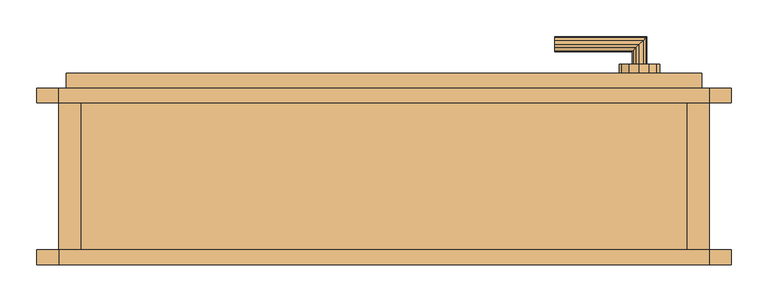
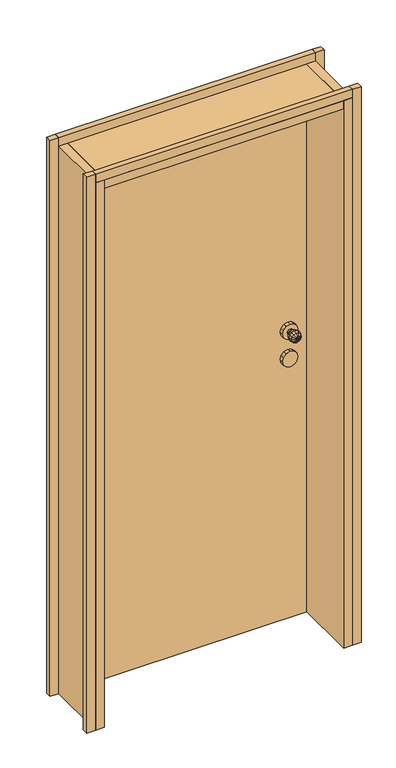
"""IFC4 building model written with IfcOpenShell, lengths in millimetres: door geometry, Tür."""

from ifc_helpers import new_model, si_unit, frame, origin, place, context, project, spatial, polyline, outline, extrude, faceted_brep, source, transform, mapped, element, save


def door_29abe8a6(model_context):
    return source(origin(), model_context, "Body", "SolidModel", [
        extrude(outline(polyline([(885.0, 220.0), (885.0, -20.0), (855.0, -20.0), (855.0, 220.0), (885.0, 220.0)])), frame((0.0, 0.0, 140.0), z_axis=(0.0, 0.0, 1.0), x_axis=(1.0, 0.0, 0.0)), (0.0, 0.0, 1.0), 1995.0),
        extrude(outline(polyline([(1176.25, 813.8156986), (1190.0, 817.5), (1203.75, 813.8156986), (1213.8156986, 803.75), (1217.5, 790.0), (1213.8156986, 776.25), (1203.75, 766.1843014), (1190.0, 762.5), (1176.25, 766.1843014), (1166.1843014, 776.25), (1162.5, 790.0), (1166.1843014, 803.75), (1176.25, 813.8156986)])), frame((0.0, 187.5, 0.0), z_axis=(0.0, 1.0, 0.0), x_axis=(0.0, 0.0, 1.0)), (0.0, 0.0, 1.0), 12.5),
        faceted_brep([(807.3205081, 150.0, 1190.0), (810.0, 160.0, 1190.0), (807.3205081, 160.0, 1200.0), (805.0, 150.0, 1198.660254), (800.0, 160.0, 1207.3205081), (798.660254, 150.0, 1205.0), (790.0, 160.0, 1210.0), (790.0, 150.0, 1207.3205081), (780.0, 160.0, 1207.3205081), (781.339746, 150.0, 1205.0), (772.6794919, 160.0, 1200.0), (775.0, 150.0, 1198.660254), (770.0, 160.0, 1190.0), (772.6794919, 150.0, 1190.0), (772.6794919, 160.0, 1180.0), (775.0, 150.0, 1181.339746), (780.0, 160.0, 1172.6794919), (781.339746, 150.0, 1175.0), (790.0, 160.0, 1170.0), (790.0, 150.0, 1172.6794919), (800.0, 160.0, 1172.6794919), (798.660254, 150.0, 1175.0), (807.3205081, 160.0, 1180.0), (805.0, 150.0, 1181.339746), (800.0, 142.6794919, 1190.0), (798.660254, 142.6794919, 1195.0), (795.0, 142.6794919, 1198.660254), (790.0, 142.6794919, 1200.0), (785.0, 142.6794919, 1198.660254), (781.339746, 142.6794919, 1195.0), (780.0, 142.6794919, 1190.0), (781.339746, 142.6794919, 1185.0), (785.0, 142.6794919, 1181.339746), (790.0, 142.6794919, 1180.0), (795.0, 142.6794919, 1181.339746), (798.660254, 142.6794919, 1185.0), (790.0, 140.0, 1190.0), (807.3205081, 170.0, 1190.0), (805.0, 170.0, 1198.660254), (798.660254, 170.0, 1205.0), (790.0, 170.0, 1207.3205081), (781.339746, 170.0, 1205.0), (775.0, 170.0, 1198.660254), (772.6794919, 170.0, 1190.0), (775.0, 170.0, 1181.339746), (781.339746, 170.0, 1175.0), (790.0, 170.0, 1172.6794919), (798.660254, 170.0, 1175.0), (805.0, 170.0, 1181.339746), (800.0, 177.3205081, 1190.0), (798.660254, 177.3205081, 1195.0), (795.0, 177.3205081, 1198.660254), (790.0, 177.3205081, 1200.0), (785.0, 177.3205081, 1198.660254), (781.339746, 177.3205081, 1195.0), (780.0, 177.3205081, 1190.0), (781.339746, 177.3205081, 1185.0), (785.0, 177.3205081, 1181.339746), (790.0, 177.3205081, 1180.0), (795.0, 177.3205081, 1181.339746), (798.660254, 177.3205081, 1185.0), (790.0, 180.0, 1190.0)], [[[0, 1, 2, 3]], [[3, 2, 4, 5]], [[5, 4, 6, 7]], [[7, 6, 8, 9]], [[9, 8, 10, 11]], [[11, 10, 12, 13]], [[13, 12, 14, 15]], [[15, 14, 16, 17]], [[17, 16, 18, 19]], [[19, 18, 20, 21]], [[21, 20, 22, 23]], [[23, 22, 1, 0]], [[24, 0, 3, 25]], [[25, 3, 5, 26]], [[26, 5, 7, 27]], [[27, 7, 9, 28]], [[28, 9, 11, 29]], [[29, 11, 13, 30]], [[30, 13, 15, 31]], [[31, 15, 17, 32]], [[32, 17, 19, 33]], [[33, 19, 21, 34]], [[34, 21, 23, 35]], [[35, 23, 0, 24]], [[36, 24, 25]], [[36, 25, 26]], [[36, 26, 27]], [[36, 27, 28]], [[36, 28, 29]], [[36, 29, 30]], [[36, 30, 31]], [[36, 31, 32]], [[36, 32, 33]], [[36, 33, 34]], [[36, 34, 35]], [[36, 35, 24]], [[1, 37, 38, 2]], [[2, 38, 39, 4]], [[4, 39, 40, 6]], [[6, 40, 41, 8]], [[8, 41, 42, 10]], [[10, 42, 43, 12]], [[12, 43, 44, 14]], [[14, 44, 45, 16]], [[16, 45, 46, 18]], [[18, 46, 47, 20]], [[20, 47, 48, 22]], [[22, 48, 37, 1]], [[37, 49, 50, 38]], [[38, 50, 51, 39]], [[39, 51, 52, 40]], [[40, 52, 53, 41]], [[41, 53, 54, 42]], [[42, 54, 55, 43]], [[43, 55, 56, 44]], [[44, 56, 57, 45]], [[45, 57, 58, 46]], [[46, 58, 59, 47]], [[47, 59, 60, 48]], [[48, 60, 49, 37]], [[49, 61, 50]], [[50, 61, 51]], [[51, 61, 52]], [[52, 61, 53]], [[53, 61, 54]], [[54, 61, 55]], [[55, 61, 56]], [[56, 61, 57]], [[57, 61, 58]], [[58, 61, 59]], [[59, 61, 60]], [[60, 61, 49]]]),
        extrude(outline(polyline([(1185.0, 798.660254), (1190.0, 800.0), (1195.0, 798.660254), (1198.660254, 795.0), (1200.0, 790.0), (1198.660254, 785.0), (1195.0, 781.339746), (1190.0, 780.0), (1185.0, 781.339746), (1181.339746, 785.0), (1180.0, 790.0), (1181.339746, 795.0), (1185.0, 798.660254)])), frame((0.0, 160.0, 0.0), z_axis=(0.0, 1.0, 0.0), x_axis=(0.0, 0.0, 1.0)), (0.0, 0.0, 1.0), 40.0),
        extrude(outline(polyline([(1066.1843014, 803.75), (1076.25, 813.8156986), (1090.0, 817.5), (1103.75, 813.8156986), (1113.8156986, 803.75), (1117.5, 790.0), (1113.8156986, 776.25), (1103.75, 766.1843014), (1090.0, 762.5), (1076.25, 766.1843014), (1066.1843014, 776.25), (1062.5, 790.0), (1066.1843014, 803.75)])), frame((0.0, 240.0, 0.0), z_axis=(0.0, 1.0, 0.0), x_axis=(0.0, 0.0, 1.0)), (0.0, 0.0, 1.0), 12.5),
        extrude(outline(polyline([(1076.25, 813.8156986), (1090.0, 817.5), (1103.75, 813.8156986), (1113.8156986, 803.75), (1117.5, 790.0), (1113.8156986, 776.25), (1103.75, 766.1843014), (1090.0, 762.5), (1076.25, 766.1843014), (1066.1843014, 776.25), (1062.5, 790.0), (1066.1843014, 803.75), (1076.25, 813.8156986)])), frame((0.0, 187.5, 0.0), z_axis=(0.0, 1.0, 0.0), x_axis=(0.0, 0.0, 1.0)), (0.0, 0.0, 1.0), 12.5),
        extrude(outline(polyline([(885.0, 220.0), (885.0, 200.0), (0.0, 200.0), (0.0, 220.0), (885.0, 220.0)])), frame((0.0, 0.0, 2135.0), z_axis=(0.0, 0.0, 1.0), x_axis=(1.0, 0.0, 0.0)), (0.0, 0.0, 1.0), 30.0),
        extrude(outline(polyline([(0.0, -20.0), (-30.0, -20.0), (-30.0, 0.0), (0.0, 0.0), (0.0, -20.0)])), frame((0.0, 0.0, 140.0), z_axis=(0.0, 0.0, 1.0), x_axis=(1.0, 0.0, 0.0)), (0.0, 0.0, 1.0), 2025.0),
        extrude(outline(polyline([(885.0, 0.0), (885.0, -20.0), (0.0, -20.0), (0.0, 0.0), (885.0, 0.0)])), frame((0.0, 0.0, 2135.0), z_axis=(0.0, 0.0, 1.0), x_axis=(1.0, 0.0, 0.0)), (0.0, 0.0, 1.0), 30.0),
        extrude(outline(polyline([(1166.1843014, 803.75), (1176.25, 813.8156986), (1190.0, 817.5), (1203.75, 813.8156986), (1213.8156986, 803.75), (1217.5, 790.0), (1213.8156986, 776.25), (1203.75, 766.1843014), (1190.0, 762.5), (1176.25, 766.1843014), (1166.1843014, 776.25), (1162.5, 790.0), (1166.1843014, 803.75)])), frame((0.0, 240.0, 0.0), z_axis=(0.0, 1.0, 0.0), x_axis=(0.0, 0.0, 1.0)), (0.0, 0.0, 1.0), 12.5),
        faceted_brep([(795.0, 240.0, 1198.660254), (790.0, 240.0, 1200.0), (785.0, 240.0, 1198.660254), (781.339746, 240.0, 1195.0), (780.0, 240.0, 1190.0), (781.339746, 240.0, 1185.0), (785.0, 240.0, 1181.339746), (790.0, 240.0, 1180.0), (795.0, 240.0, 1181.339746), (798.660254, 240.0, 1185.0), (800.0, 240.0, 1190.0), (798.660254, 240.0, 1195.0), (790.0, 280.0, 1200.0), (795.0, 285.0, 1198.660254), (798.660254, 288.660254, 1195.0), (800.0, 290.0, 1190.0), (798.660254, 288.660254, 1185.0), (795.0, 285.0, 1181.339746), (790.0, 280.0, 1180.0), (785.0, 275.0, 1181.339746), (781.339746, 271.339746, 1185.0), (780.0, 270.0, 1190.0), (781.339746, 271.339746, 1195.0), (785.0, 275.0, 1198.660254), (675.0, 275.0, 1198.660254), (675.0, 280.0, 1200.0), (675.0, 285.0, 1198.660254), (675.0, 288.660254, 1195.0), (675.0, 290.0, 1190.0), (675.0, 288.660254, 1185.0), (675.0, 285.0, 1181.339746), (675.0, 280.0, 1180.0), (675.0, 275.0, 1181.339746), (675.0, 271.339746, 1185.0), (675.0, 270.0, 1190.0), (675.0, 271.339746, 1195.0)], [[[0, 1, 2, 3, 4, 5, 6, 7, 8, 9, 10, 11]], [[12, 1, 0, 13]], [[13, 0, 11, 14]], [[14, 11, 10, 15]], [[15, 10, 9, 16]], [[16, 9, 8, 17]], [[17, 8, 7, 18]], [[18, 7, 6, 19]], [[19, 6, 5, 20]], [[20, 5, 4, 21]], [[21, 4, 3, 22]], [[22, 3, 2, 23]], [[23, 2, 1, 12]], [[24, 25, 26, 27, 28, 29, 30, 31, 32, 33, 34, 35]], [[25, 12, 13, 26]], [[26, 13, 14, 27]], [[27, 14, 15, 28]], [[28, 15, 16, 29]], [[29, 16, 17, 30]], [[30, 17, 18, 31]], [[31, 18, 19, 32]], [[32, 19, 20, 33]], [[33, 20, 21, 34]], [[34, 21, 22, 35]], [[35, 22, 23, 24]], [[24, 23, 12, 25]]]),
        extrude(outline(polyline([(30.0, 220.0), (30.0, -20.0), (0.0, -20.0), (0.0, 220.0), (30.0, 220.0)])), frame((0.0, 0.0, 140.0), z_axis=(0.0, 0.0, 1.0), x_axis=(1.0, 0.0, 0.0)), (0.0, 0.0, 1.0), 1995.0),
        extrude(outline(polyline([(0.0, 200.0), (-30.0, 200.0), (-30.0, 220.0), (0.0, 220.0), (0.0, 200.0)])), frame((0.0, 0.0, 140.0), z_axis=(0.0, 0.0, 1.0), x_axis=(1.0, 0.0, 0.0)), (0.0, 0.0, 1.0), 2025.0),
        extrude(outline(polyline([(915.0, 220.0), (915.0, 200.0), (885.0, 200.0), (885.0, 220.0), (915.0, 220.0)])), frame((0.0, 0.0, 140.0), z_axis=(0.0, 0.0, 1.0), x_axis=(1.0, 0.0, 0.0)), (0.0, 0.0, 1.0), 2025.0),
        extrude(outline(polyline([(915.0, 0.0), (915.0, -20.0), (885.0, -20.0), (885.0, 0.0), (915.0, 0.0)])), frame((0.0, 0.0, 140.0), z_axis=(0.0, 0.0, 1.0), x_axis=(1.0, 0.0, 0.0)), (0.0, 0.0, 1.0), 2025.0),
        extrude(outline(polyline([(875.0, 240.0), (875.0, 200.0), (10.0, 200.0), (10.0, 240.0), (875.0, 240.0)])), frame((0.0, 0.0, 140.0), z_axis=(0.0, 0.0, 1.0), x_axis=(1.0, 0.0, 0.0)), (0.0, 0.0, 1.0), 1985.0),
        extrude(outline(polyline([(855.0, 220.0), (855.0, -20.0), (30.0, -20.0), (30.0, 220.0), (855.0, 220.0)])), frame((0.0, 0.0, 2105.0), z_axis=(0.0, 0.0, 1.0), x_axis=(1.0, 0.0, 0.0)), (0.0, 0.0, 1.0), 30.0),
    ])


if __name__ == "__main__":
    model = new_model("IFC4")
    model_context = context("Model", 3, world=origin())
    ifc_project = project(units=[si_unit("LENGTHUNIT", "METRE", prefix="MILLI")], contexts=[model_context])
    site = spatial("IfcSite", under=ifc_project)
    building = spatial("IfcBuilding", under=site)
    placement = place(None, origin())
    door_shape = door_29abe8a6(model_context)
    element("IfcDoor", 1, ObjectType="Tür", at=placement, inside=building, context=model_context, shape_type="MappedRepresentation", body=[
        mapped(door_shape, transform((0.0, 0.0, 0.0), x_axis=(1.0, 0.0, 0.0), y_axis=(0.0, 1.0, 0.0), z_axis=(0.0, 0.0, 1.0))),
    ])
    save(model, "model.ifc")

# Revit data of these elements
# Type "Tür"
#   Type Mark = "65"
# Element 1 (IfcDoor, "Tür")
#   Materials on its faces: "Entwcol-Glas-Typ1"
# Materials
#   "Entwcol-Glas-Typ1": class "Unassigned", colour RGB 128 128 128, transparency 0.55
